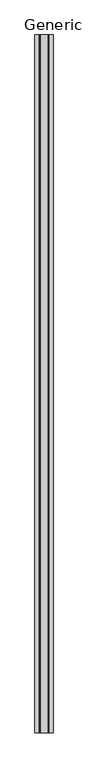
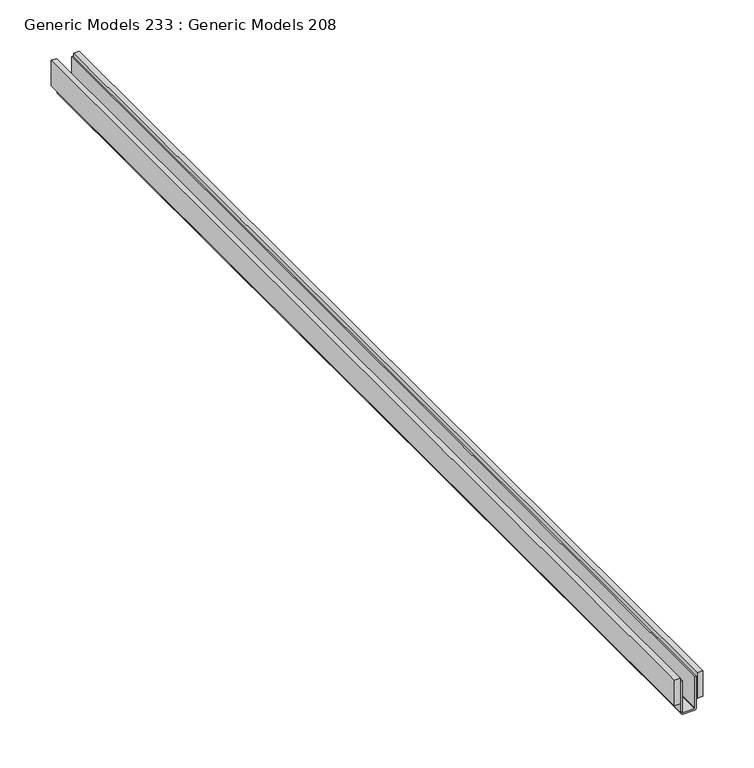
"""IFC4 building model written with IfcOpenShell, lengths in millimetres: proxy geometry, Generic Models 233 : Generic Models 208."""

from ifc_helpers import new_model, si_unit, point, frame, frame_2d, origin, place, context, project, spatial, polyline, circle_curve, trimmed, segment, composite_curve, outline, extrude, source, transform, mapped, element, save


def generic_models_233_generic_models_208_18d11060(model_context):
    return source(origin(), model_context, "Body", "SweptSolid", [
        extrude(outline(polyline([(53933.2396911, 990.4966182), (53939.5896911, 990.4966182), (53939.5896911, -228.7033818), (53933.2396911, -228.7033818), (53933.2396911, 990.4966182)])), frame((0.0, 0.0, 1971.2519616), z_axis=(0.0, 0.0, 1.0), x_axis=(1.0, 0.0, 0.0)), (0.0, 0.0, 1.0), 30.1625),
        extrude(outline(composite_curve([segment(trimmed(circle_curve(frame_2d((1960.1213761, 53942.7466056)), 2.3631645), [point((1960.1213761, 53940.3834411))], [point((1957.7582116, 53942.7466056))], False, "CARTESIAN"), True, "CONTINUOUS"), segment(polyline([(1957.7582116, 53942.7466056), (1957.7582116, 53955.4662341)]), True, "CONTINUOUS"), segment(trimmed(circle_curve(frame_2d((1960.1379186, 53955.4662341)), 2.379707), [point((1957.7582116, 53955.4662341))], [point((1960.1379186, 53957.8459411))], False, "CARTESIAN"), True, "CONTINUOUS"), segment(polyline([(1960.1379186, 53957.8459411), (1997.6441491, 53957.8459411), (1997.6441491, 53956.2584411), (1960.1379186, 53956.2584411)]), True, "CONTINUOUS"), segment(trimmed(circle_curve(frame_2d((1960.1379186, 53955.4662341)), 0.792207), [point((1960.1379186, 53956.2584411))], [point((1959.3457116, 53955.4662341))], True, "CARTESIAN"), True, "CONTINUOUS"), segment(polyline([(1959.3457116, 53955.4662341), (1959.3457116, 53942.7466056)]), True, "CONTINUOUS"), segment(trimmed(circle_curve(frame_2d((1960.1213761, 53942.7466056)), 0.7756645), [point((1959.3457116, 53942.7466056))], [point((1960.1213761, 53941.9709411))], True, "CARTESIAN"), True, "CONTINUOUS"), segment(polyline([(1960.1213761, 53941.9709411), (1997.6441491, 53941.9709411), (1997.6441491, 53940.3834411), (1960.1213761, 53940.3834411)]), True, "CONTINUOUS")], self_intersect=False)), frame((0.0, -228.7033818, 0.0), z_axis=(0.0, 1.0, 0.0), x_axis=(0.0, 0.0, 1.0)), (0.0, 0.0, 1.0), 1219.2),
        extrude(outline(polyline([(53958.6396911, 990.4966182), (53964.9896911, 990.4966182), (53964.9896911, -228.7033818), (53958.6396911, -228.7033818), (53958.6396911, 990.4966182)])), frame((0.0, 0.0, 1971.2519616), z_axis=(0.0, 0.0, 1.0), x_axis=(1.0, 0.0, 0.0)), (0.0, 0.0, 1.0), 30.1625),
    ])


if __name__ == "__main__":
    model = new_model("IFC4")
    model_context = context("Model", 3, world=origin())
    ifc_project = project(units=[si_unit("LENGTHUNIT", "METRE", prefix="MILLI")], contexts=[model_context])
    site = spatial("IfcSite", under=ifc_project)
    building = spatial("IfcBuilding", under=site)
    placement = place(None, origin())
    generic_models_233_generic_models_208_shape = generic_models_233_generic_models_208_18d11060(model_context)
    element("IfcBuildingElementProxy", 1, Name="Generic Models 233 : Generic Models 208", ObjectType="Generic Models 233 : Generic Models 208", at=placement, inside=building, context=model_context, shape_type="MappedRepresentation", body=[
        mapped(generic_models_233_generic_models_208_shape, transform((0.0, 0.0, 0.0), x_axis=(1.0, 0.0, 0.0), y_axis=(0.0, 1.0, 0.0), z_axis=(0.0, 0.0, 1.0))),
    ])
    save(model, "model.ifc")
